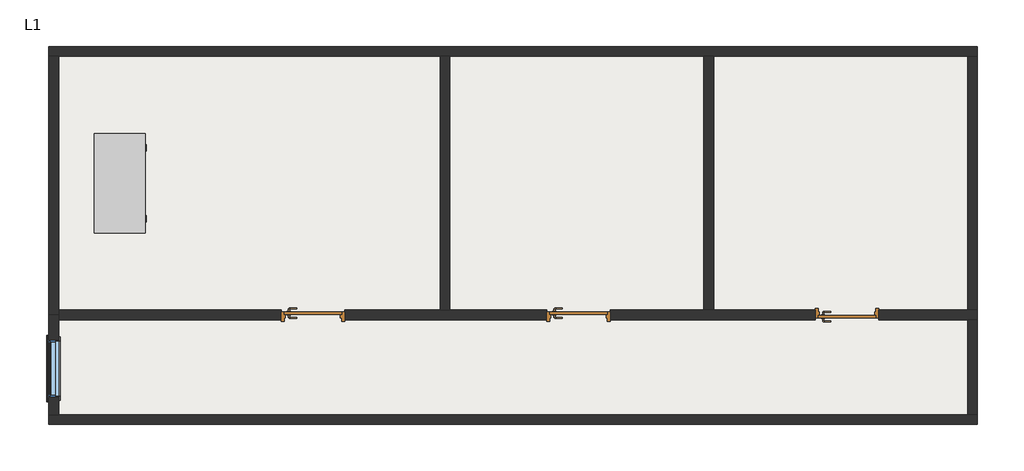
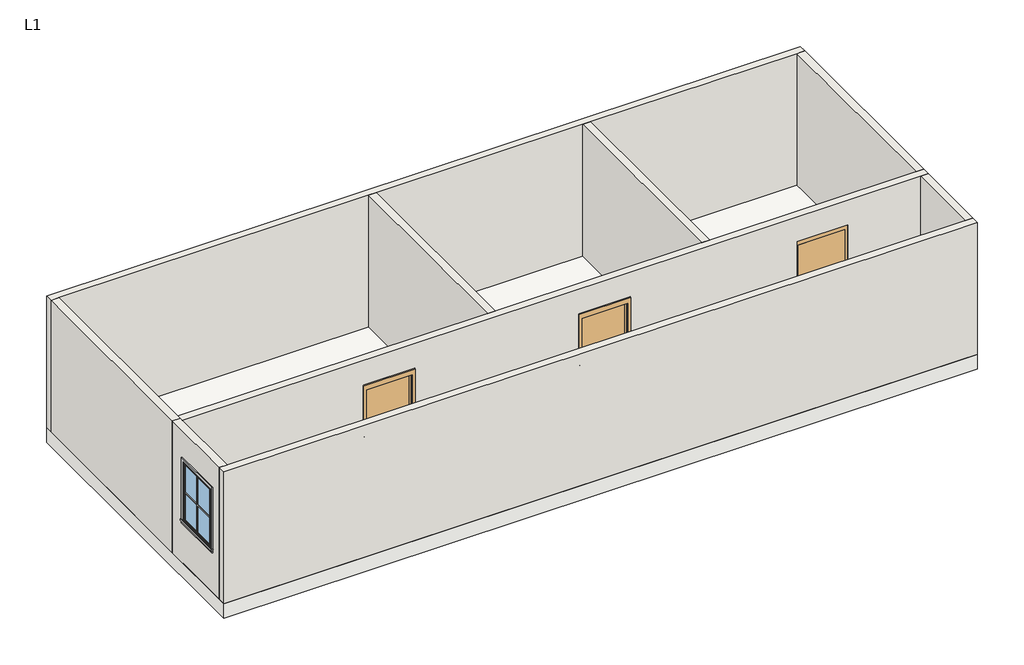
# One storey: 9 walls, 3 doors, 3 proxies, 1 furniture element, 1 slab, 1 window.
"""IFC4 building model written with IfcOpenShell, lengths in millimetres."""

import ifcopenshell
import ifcopenshell.guid

model = None  # the IFC model being written
_history = None  # IfcOwnerHistory: only IFC2X3 demands one
_inside = {}  # id of a spatial element -> (the spatial element, [elements in it])
_under = {}  # id of a project, library or spatial element -> (it, [spatial elements below it])
_declared = {}  # id of a project -> (the project, [libraries it declares])
_typed = {}  # id of a type object -> (the type object, [elements of that type])
_made_of = {}  # id of a material, layer set ... -> (it, [elements and type objects made of it])


def new_model(schema):
    """Start an empty IFC model of exactly this schema.

    Asked for "IFC4X3", IfcOpenShell would pick the latest addendum, in which some entities
    have other attributes; the version numbers below select the first issue.
    IFC2X3 requires an IfcOwnerHistory on every rooted entity: one is made here for all.
    """
    global model, _history
    if schema == "IFC4X3":
        model = ifcopenshell.file(schema_version=(4, 3, 0, 0))
    else:
        model = ifcopenshell.file(schema=schema)
    _inside.clear()
    _under.clear()
    _declared.clear()
    _typed.clear()
    _made_of.clear()
    _history = None
    if model.schema == "IFC2X3":
        org = make("IfcOrganization", Name="unknown")
        user = make(
            "IfcPersonAndOrganization",
            ThePerson=make("IfcPerson", FamilyName="unknown"),
            TheOrganization=org,
        )
        app = make(
            "IfcApplication",
            ApplicationDeveloper=org,
            Version="unknown",
            ApplicationFullName="unknown",
            ApplicationIdentifier="unknown",
        )
        _history = make(
            "IfcOwnerHistory",
            OwningUser=user,
            OwningApplication=app,
            ChangeAction="ADDED",
            CreationDate=0,
        )
    return model


def make(cls, **values):
    """One entity of the class cls with the attributes given. An attribute that is None is left unset."""
    return model.create_entity(
        cls, **{name: value for name, value in values.items() if value is not None}
    )


def rooted(cls, **values):
    """An entity with a GlobalId (a new one), such as an element, a storey or a relation."""
    return make(cls, GlobalId=ifcopenshell.guid.new(), OwnerHistory=_history, **values)


def si_unit(unit_type, name, prefix=None):
    """IfcSIUnit, for example si_unit("LENGTHUNIT", "METRE", prefix="MILLI")."""
    return make("IfcSIUnit", UnitType=unit_type, Prefix=prefix, Name=name)


def assignment(units):
    """IfcUnitAssignment: the units of a project."""
    return None if units is None else make("IfcUnitAssignment", Units=units)


def point(xyz):
    """IfcCartesianPoint."""
    return None if xyz is None else make("IfcCartesianPoint", Coordinates=xyz)


def direction(xyz):
    """IfcDirection."""
    return None if xyz is None else make("IfcDirection", DirectionRatios=xyz)


def frame(location, z_axis=None, x_axis=None):
    """IfcAxis2Placement3D, a coordinate frame: its origin and axes. An axis left out is left unset."""
    return make(
        "IfcAxis2Placement3D",
        Location=point(location),
        Axis=direction(z_axis),
        RefDirection=direction(x_axis),
    )


def frame_2d(location, x_axis=None):
    """IfcAxis2Placement2D, a coordinate frame in the plane: its origin and x axis."""
    return make(
        "IfcAxis2Placement2D", Location=point(location), RefDirection=direction(x_axis)
    )


def origin():
    """The frame at (0, 0, 0) with its axes left unset."""
    return frame((0.0, 0.0, 0.0))


def origin_with_axes():
    """The frame at (0, 0, 0) with the z axis (0, 0, 1) and the x axis (1, 0, 0) written out."""
    return frame((0.0, 0.0, 0.0), z_axis=(0.0, 0.0, 1.0), x_axis=(1.0, 0.0, 0.0))


def place(relative_to, where):
    """IfcLocalPlacement: puts the frame where relative to a parent placement (None: the world)."""
    return make(
        "IfcLocalPlacement", PlacementRelTo=relative_to, RelativePlacement=where
    )


def context(
    kind, dimensions, precision=None, world=None, true_north=None, identifier=None
):
    """IfcGeometricRepresentationContext, for example the 3D "Model" context."""
    return make(
        "IfcGeometricRepresentationContext",
        ContextIdentifier=identifier,
        ContextType=kind,
        CoordinateSpaceDimension=dimensions,
        Precision=precision,
        WorldCoordinateSystem=world,
        TrueNorth=true_north,
    )


def project(units=None, contexts=None):
    """IfcProject with its units and contexts."""
    return rooted(
        "IfcProject",
        Name="project",
        RepresentationContexts=contexts,
        UnitsInContext=assignment(units),
    )


def spatial(cls, under=None, at=None, **own):
    """A site, building, storey or space (cls), placed at a placement, below another one or the project."""
    s = rooted(cls, ObjectPlacement=at, **own)
    if under is not None:
        _under.setdefault(under.id(), (under, []))[1].append(s)
    return s


def polyline(points):
    """IfcPolyline through the points."""
    return make("IfcPolyline", Points=[point(p) for p in points])


def circle_curve(where, radius):
    """IfcCircle in the frame where."""
    return make("IfcCircle", Position=where, Radius=radius)


def ellipse_curve(where, semi_axis1, semi_axis2):
    """IfcEllipse in the frame where."""
    return make(
        "IfcEllipse", Position=where, SemiAxis1=semi_axis1, SemiAxis2=semi_axis2
    )


def trimmed(basis, trim1, trim2, sense, master):
    """IfcTrimmedCurve: the piece of a basis curve between two trims."""
    return make(
        "IfcTrimmedCurve",
        BasisCurve=basis,
        Trim1=trim1,
        Trim2=trim2,
        SenseAgreement=sense,
        MasterRepresentation=master,
    )


def segment(curve, same_sense, transition):
    """IfcCompositeCurveSegment."""
    return make(
        "IfcCompositeCurveSegment",
        Transition=transition,
        SameSense=same_sense,
        ParentCurve=curve,
    )


def composite_curve(segments, self_intersect=None):
    """IfcCompositeCurve: segments joined end to end."""
    return make("IfcCompositeCurve", Segments=segments, SelfIntersect=self_intersect)


def outline(outer, holes=None, kind="AREA"):
    """IfcArbitraryClosedProfileDef: a profile drawn as a closed curve; with holes, ...WithVoids."""
    if holes is None:
        return make("IfcArbitraryClosedProfileDef", ProfileType=kind, OuterCurve=outer)
    return make(
        "IfcArbitraryProfileDefWithVoids",
        ProfileType=kind,
        OuterCurve=outer,
        InnerCurves=holes,
    )


def extrude(swept, where, along, depth):
    """IfcExtrudedAreaSolid: the profile swept, set in the frame where, extruded along a direction by depth."""
    return make(
        "IfcExtrudedAreaSolid",
        SweptArea=swept,
        Position=where,
        ExtrudedDirection=direction(along),
        Depth=depth,
    )


def faces_of(points, faces, orient=None, outer=None):
    """IfcFace entities. A face is a list of loops; a loop is a list of indices into points, from 0.

    orient and outer hold one flag for each loop. By default every Orientation is true, the
    first loop of a face is its IfcFaceOuterBound and the others are IfcFaceBound.
    """
    made = []
    for i, loops in enumerate(faces):
        bounds = []
        for j, loop in enumerate(loops):
            is_outer = j == 0 if outer is None else outer[i][j]
            bounds.append(
                make(
                    "IfcFaceOuterBound" if is_outer else "IfcFaceBound",
                    Bound=make("IfcPolyLoop", Polygon=[points[k] for k in loop]),
                    Orientation=True if orient is None else orient[i][j],
                )
            )
        made.append(make("IfcFace", Bounds=bounds))
    return made


def faceted_brep(points, faces, orient=None, outer=None, voids=None):
    """IfcFacetedBrep: a solid bounded by flat faces; with voids (closed shells), ...WithVoids."""
    shared = [point(p) for p in points]
    hull = make("IfcClosedShell", CfsFaces=faces_of(shared, faces, orient, outer))
    if voids is None:
        return make("IfcFacetedBrep", Outer=hull)
    return make(
        "IfcFacetedBrepWithVoids",
        Outer=hull,
        Voids=[
            make(cls, CfsFaces=faces_of(shared, fs, o, b)) for cls, fs, o, b in voids
        ],
    )


def shape(context_of_items, identifier, shape_type, items):
    """IfcShapeRepresentation: the items that make up one representation, for example the "Body"."""
    return make(
        "IfcShapeRepresentation",
        ContextOfItems=context_of_items,
        RepresentationIdentifier=identifier,
        RepresentationType=shape_type,
        Items=items,
    )


def source(mapping_origin, context_of_items, identifier, shape_type, items):
    """IfcRepresentationMap: a shape defined once, which mapped items show again and again."""
    return make(
        "IfcRepresentationMap",
        MappingOrigin=mapping_origin,
        MappedRepresentation=shape(context_of_items, identifier, shape_type, items),
    )


def transform(
    local_origin,
    x_axis=None,
    y_axis=None,
    z_axis=None,
    scale=None,
    scale2=None,
    scale3=None,
    uniform=True,
):
    """IfcCartesianTransformationOperator3D, or its non-uniform kind. x_axis, y_axis, z_axis: its Axis1, 2, 3."""
    if uniform:
        return make(
            "IfcCartesianTransformationOperator3D",
            Axis1=direction(x_axis),
            Axis2=direction(y_axis),
            LocalOrigin=point(local_origin),
            Scale=scale,
            Axis3=direction(z_axis),
        )
    return make(
        "IfcCartesianTransformationOperator3DnonUniform",
        Axis1=direction(x_axis),
        Axis2=direction(y_axis),
        LocalOrigin=point(local_origin),
        Scale=scale,
        Axis3=direction(z_axis),
        Scale2=scale2,
        Scale3=scale3,
    )


def mapped(mapping_source, mapping_target):
    """IfcMappedItem: shows the shape of a source again, moved by a transform."""
    return make(
        "IfcMappedItem", MappingSource=mapping_source, MappingTarget=mapping_target
    )


def made_of(thing, what):
    """Note that an element or type object is made of a material, layer set ...; save() writes the relation."""
    if what is not None:
        _made_of.setdefault(what.id(), (what, []))[1].append(thing)
    return thing


def element(
    cls,
    number,
    at=None,
    inside=None,
    cuts=None,
    type_object=None,
    material=None,
    context=None,
    identifier="Body",
    shape_type=None,
    held_by="IfcProductDefinitionShape",
    body=None,
    shapes=None,
    **own,
):
    """One element of the class cls, such as IfcWall. Its Tag is "e" and its number.

    at: its placement. inside: the storey or other place that contains it. cuts: it is an
    opening in that element (IfcRelVoidsElement). A single representation is given by context,
    identifier, shape_type and body (its items); several are given by shapes. held_by: the class
    of the entity that holds the representations. save() writes the other relations.
    """
    e = rooted(cls, Tag="e%d" % number, ObjectPlacement=at, **own)
    if body is not None:
        shapes = [shape(context, identifier, shape_type, body)]
    if shapes is not None:
        e.Representation = make(held_by, Representations=shapes)
    if inside is not None:
        _inside.setdefault(inside.id(), (inside, []))[1].append(e)
    if cuts is not None:
        rooted(
            "IfcRelVoidsElement", RelatingBuildingElement=cuts, RelatedOpeningElement=e
        )
    if type_object is not None:
        _typed.setdefault(type_object.id(), (type_object, []))[1].append(e)
    return made_of(e, material)


def aggregate(whole, parts):
    """IfcRelAggregates: a whole, such as a stair, and the parts it consists of."""
    return rooted("IfcRelAggregates", RelatingObject=whole, RelatedObjects=parts)


def save(model, path):
    """Write the relations noted so far, then the file.

    IfcRelAggregates (storeys below a building ...), IfcRelContainedInSpatialStructure (elements
    in a storey), IfcRelDefinesByType, IfcRelAssociatesMaterial and IfcRelDeclares: one each for
    every whole, place, type object, material and project.
    """
    for whole, parts in _under.values():
        aggregate(whole, parts)
    for where, things in _inside.values():
        rooted(
            "IfcRelContainedInSpatialStructure",
            RelatedElements=things,
            RelatingStructure=where,
        )
    for kind, things in _typed.values():
        rooted("IfcRelDefinesByType", RelatedObjects=things, RelatingType=kind)
    for what, things in _made_of.values():
        rooted("IfcRelAssociatesMaterial", RelatedObjects=things, RelatingMaterial=what)
    for by, libraries in _declared.values():
        rooted("IfcRelDeclares", RelatingContext=by, RelatedDefinitions=libraries)
    model.write(path)


def plane_surface(at):
    """IfcPlane: the flat surface through the origin of the frame at, square to its z axis."""
    return make("IfcPlane", Position=at)


def cylinder_surface(at, radius):
    """IfcCylindricalSurface: all points at the distance radius from the z axis of the frame at."""
    return make("IfcCylindricalSurface", Position=at, Radius=radius)


def revolved_surface(curve, axis_point, axis_direction):
    """IfcSurfaceOfRevolution: the curve turned about the line through axis_point along axis_direction."""
    return make(
        "IfcSurfaceOfRevolution",
        SweptCurve=make("IfcArbitraryOpenProfileDef", ProfileType="CURVE", Curve=curve),
        AxisPosition=make("IfcAxis1Placement", Location=point(axis_point), Axis=direction(axis_direction)),
    )


def advanced_brep(points, edges, surfaces, faces):
    """IfcAdvancedBrep: a solid bounded by faces that lie on surfaces and meet in shared edges.

    An edge is (start, end): straight between two places in points (the first is 0);
    or (start, end, curve); or (start, end, curve, False) where it runs against its curve.
    A face is (place in surfaces, loops), or (place, loops, False) where it looks against
    its surface's normal. A loop lists edges by number (the first is 1), with a minus sign
    where the edge is run from its end to its start. The first loop is the outer one.
    """
    corners = [point(p) for p in points]
    vertices = [make("IfcVertexPoint", VertexGeometry=c) for c in corners]
    made = []
    for start, end, *more in edges:
        made.append(
            make(
                "IfcEdgeCurve",
                EdgeStart=vertices[start],
                EdgeEnd=vertices[end],
                EdgeGeometry=more[0] if more else make("IfcPolyline", Points=[corners[start], corners[end]]),
                SameSense=more[1] if len(more) > 1 else True,
            )
        )
    hull = []
    for where, loops, *sense in faces:
        bounds = []
        for j, loop in enumerate(loops):
            ring = [make("IfcOrientedEdge", EdgeElement=made[abs(k) - 1], Orientation=k > 0) for k in loop]
            bounds.append(
                make(
                    "IfcFaceOuterBound" if j == 0 else "IfcFaceBound",
                    Bound=make("IfcEdgeLoop", EdgeList=ring),
                    Orientation=True,
                )
            )
        hull.append(make("IfcAdvancedFace", Bounds=bounds, FaceSurface=surfaces[where], SameSense=sense[0] if sense else True))
    return make("IfcAdvancedBrep", Outer=make("IfcClosedShell", CfsFaces=hull))


def m_muntin_pattern_2x2_m_muntin_pattern_2x2_ad852c99(model_context):
    return source(origin(), model_context, "Body", "SweptSolid", [
        extrude(outline(polyline([(568.25, -6.35), (568.25, -411.9), (555.55, -411.9), (555.55, -6.35), (0.0, -6.35), (0.0, 6.35), (555.55, 6.35), (555.55, 411.9), (568.25, 411.9), (568.25, 6.35), (1123.8, 6.35), (1123.8, -6.35), (568.25, -6.35)])), frame((0.0, -22.225, 0.0), z_axis=(0.0, 1.0, 0.0), x_axis=(0.0, 0.0, 1.0)), (0.0, 0.0, 1.0), 12.7),
        extrude(outline(polyline([(568.25, -6.35), (568.25, -411.9), (555.55, -411.9), (555.55, -6.35), (0.0, -6.35), (0.0, 6.35), (555.55, 6.35), (555.55, 411.9), (568.25, 411.9), (568.25, 6.35), (1123.8, 6.35), (1123.8, -6.35), (568.25, -6.35)])), frame((0.0, 9.525, 0.0), z_axis=(0.0, 1.0, 0.0), x_axis=(0.0, 0.0, 1.0)), (0.0, 0.0, 1.0), 12.7),
    ])


def m_trim_window_exterior_flat_with_sill_71544b40(model_context):
    return source(origin(), model_context, "Body", "SweptSolid", [
        extrude(outline(polyline([(510.0, -1220.4323709), (510.0, -1280.4323709), (-510.0, -1280.4323709), (-510.0, -1220.4323709), (510.0, -1220.4323709)])), origin_with_axes(), (0.0, 0.0, 1.0), 19.05),
        extrude(outline(polyline([(-1230.0, 38.1), (-1202.4580645, 38.1), (-1200.0, 19.05), (-1200.0, 0.0), (-1220.4323709, 0.0), (-1220.4323709, 19.05), (-1230.0, 19.05), (-1230.0, 38.1)])), frame((-522.7, 0.0, 0.0), z_axis=(1.0, 0.0, 0.0), x_axis=(0.0, 1.0, 0.0)), (0.0, 0.0, 1.0), 1045.4),
        extrude(outline(polyline([(-510.0, 60.0), (510.0, 60.0), (510.0, -1200.0), (450.0, -1200.0), (450.0, 0.0), (-450.0, 0.0), (-450.0, -1200.0), (-510.0, -1200.0), (-510.0, 60.0)])), origin_with_axes(), (0.0, 0.0, 1.0), 19.05),
    ])


def m_trim_window_interior_flat_picture_frame_24fe8ef8(model_context):
    return source(origin(), model_context, "Body", "SweptSolid", [
        extrude(outline(polyline([(497.3, 47.3), (497.3, -1247.3), (-497.3, -1247.3), (-497.3, 47.3), (497.3, 47.3)]), holes=[polyline([(437.3, -12.7), (-437.3, -12.7), (-437.3, -1187.3), (437.3, -1187.3), (437.3, -12.7)])]), origin_with_axes(), (0.0, 0.0, 1.0), 30.0),
    ])


def m_door_passage_single_flush_900_x_2100mm_f70d95c9(model_context):
    return source(origin(), model_context, "Body", "SolidModel", [
        advanced_brep(
        [(-384.990625, 3.35, 1000.0), (-364.990625, 3.35, 1000.0), (-364.990625, -26.65, 1000.0), (-384.990625, -26.65, 1000.0), (-359.990625, -31.65, 1000.0), (-359.990625, -51.65, 1000.0), (-254.990625, -51.65, 1000.0), (-254.990625, -31.65, 1000.0)],
        [
            (0, 1, circle_curve(frame((-374.990625, 3.35, 1000.0), z_axis=(0.0, 1.0, 0.0), x_axis=(1.0, 0.0, 0.0)), 10.0)),
            (1, 0, circle_curve(frame((-374.990625, 3.35, 1000.0), z_axis=(0.0, 1.0, 0.0), x_axis=(1.0, 0.0, 0.0)), 10.0)),
            (1, 2),
            (2, 3, circle_curve(frame((-374.990625, -26.65, 1000.0), z_axis=(0.0, 1.0, 0.0), x_axis=(1.0, 0.0, 0.0)), 10.0)),
            (3, 0),
            (3, 2, circle_curve(frame((-374.990625, -26.65, 1000.0), z_axis=(0.0, 1.0, 0.0), x_axis=(1.0, 0.0, 0.0)), 10.0)),
            (4, 5, circle_curve(frame((-359.990625, -41.65, 1000.0), z_axis=(-1.0, 0.0, 0.0), x_axis=(0.0, 1.0, 0.0)), 10.0)),
            (5, 3, circle_curve(frame((-359.990625, -26.65, 1000.0), z_axis=(0.0, 0.0, -1.0), x_axis=(-1.0, 0.0, 0.0)), 25.0)),
            (2, 4, circle_curve(frame((-359.990625, -26.65, 1000.0), z_axis=(0.0, 0.0, 1.0), x_axis=(-1.0, 0.0, 0.0)), 5.0)),
            (5, 4, circle_curve(frame((-359.990625, -41.65, 1000.0), z_axis=(-1.0, 0.0, 0.0), x_axis=(0.0, 1.0, 0.0)), 10.0)),
            (6, 7, circle_curve(frame((-254.990625, -41.65, 1000.0), z_axis=(1.0, 0.0, 0.0), x_axis=(0.0, 1.0, 0.0)), 10.0)),
            (7, 6, circle_curve(frame((-254.990625, -41.65, 1000.0), z_axis=(1.0, 0.0, 0.0), x_axis=(0.0, 1.0, 0.0)), 10.0)),
            (4, 7),
            (6, 5),
        ],
        [
            plane_surface(frame((-374.990625, 3.35, 1000.0), z_axis=(0.0, 1.0, 0.0), x_axis=(0.0, 0.0, 1.0))),
            cylinder_surface(frame((-374.990625, 3.35, 1000.0), z_axis=(0.0, 1.0, 0.0), x_axis=(1.0, 0.0, 0.0)), 10.0),
            revolved_surface(trimmed(ellipse_curve(frame((-374.990625, -26.65, 1000.0), z_axis=(0.0, -1.0, 0.0), x_axis=(1.0, 0.0, 0.0)), 10.0, 10.0), [point((-384.990625, -26.65, 1000.0))], [point((-364.990625, -26.65, 1000.0))], True, "CARTESIAN"), (-359.990625, -26.65, 1000.0), (0.0, 0.0, -1.0)),
            revolved_surface(trimmed(ellipse_curve(frame((-374.990625, -26.65, 1000.0), z_axis=(0.0, -1.0, 0.0), x_axis=(1.0, 0.0, 0.0)), 10.0, 10.0), [point((-364.990625, -26.65, 1000.0))], [point((-384.990625, -26.65, 1000.0))], True, "CARTESIAN"), (-359.990625, -26.65, 1000.0), (0.0, 0.0, -1.0)),
            plane_surface(frame((-254.990625, -41.65, 1000.0), z_axis=(1.0, 0.0, 0.0), x_axis=(0.0, 0.0, 1.0))),
            cylinder_surface(frame((-359.990625, -41.65, 1000.0), z_axis=(-1.0, 0.0, 0.0), x_axis=(0.0, 1.0, 0.0)), 10.0),
        ],
        [
            (0, [[1, 2]]),
            (1, [[3, 4, 5, -2]]),
            (1, [[-5, 6, -3, -1]]),
            (2, [[7, 8, -4, 9]]),
            (3, [[10, -9, -6, -8]]),
            (4, [[11, 12]]),
            (5, [[13, -11, 14, -7]]),
            (5, [[-14, -12, -13, -10]]),
        ],
    ),
        extrude(outline(composite_curve([segment(trimmed(circle_curve(frame_2d((1000.0, -377.490625)), 30.0), [point((1000.0, -407.490625))], [point((1000.0, -347.490625))], False, "CARTESIAN"), True, "CONTINUOUS"), segment(trimmed(circle_curve(frame_2d((1000.0, -377.490625)), 30.0), [point((1000.0, -347.490625))], [point((1000.0, -407.490625))], False, "CARTESIAN"), True, "CONTINUOUS")], self_intersect=False)), frame((0.0, 3.35, 0.0), z_axis=(0.0, 1.0, 0.0), x_axis=(0.0, 0.0, 1.0)), (0.0, 0.0, 1.0), 8.0),
        advanced_brep(
        [(-384.990625, 64.35, 1000.0), (-364.990625, 64.35, 1000.0), (-384.990625, 94.35, 1000.0), (-364.990625, 94.35, 1000.0), (-359.990625, 99.35, 1000.0), (-359.990625, 119.35, 1000.0), (-254.990625, 119.35, 1000.0), (-254.990625, 99.35, 1000.0)],
        [
            (0, 1, circle_curve(frame((-374.990625, 64.35, 1000.0), z_axis=(0.0, -1.0, 0.0), x_axis=(1.0, 0.0, 0.0)), 10.0)),
            (1, 0, circle_curve(frame((-374.990625, 64.35, 1000.0), z_axis=(0.0, -1.0, 0.0), x_axis=(1.0, 0.0, 0.0)), 10.0)),
            (0, 2),
            (2, 3, circle_curve(frame((-374.990625, 94.35, 1000.0), z_axis=(0.0, -1.0, 0.0), x_axis=(1.0, 0.0, 0.0)), 10.0)),
            (3, 1),
            (3, 2, circle_curve(frame((-374.990625, 94.35, 1000.0), z_axis=(0.0, -1.0, 0.0), x_axis=(1.0, 0.0, 0.0)), 10.0)),
            (4, 3, circle_curve(frame((-359.990625, 94.35, 1000.0), z_axis=(0.0, 0.0, 1.0), x_axis=(-1.0, 0.0, 0.0)), 5.0)),
            (2, 5, circle_curve(frame((-359.990625, 94.35, 1000.0), z_axis=(0.0, 0.0, -1.0), x_axis=(-1.0, 0.0, 0.0)), 25.0)),
            (5, 4, circle_curve(frame((-359.990625, 109.35, 1000.0), z_axis=(-1.0, 0.0, 0.0), x_axis=(0.0, -1.0, 0.0)), 10.0)),
            (4, 5, circle_curve(frame((-359.990625, 109.35, 1000.0), z_axis=(-1.0, 0.0, 0.0), x_axis=(0.0, -1.0, 0.0)), 10.0)),
            (6, 7, circle_curve(frame((-254.990625, 109.35, 1000.0), z_axis=(1.0, 0.0, 0.0), x_axis=(0.0, -1.0, 0.0)), 10.0)),
            (7, 6, circle_curve(frame((-254.990625, 109.35, 1000.0), z_axis=(1.0, 0.0, 0.0), x_axis=(0.0, -1.0, 0.0)), 10.0)),
            (5, 6),
            (7, 4),
        ],
        [
            plane_surface(frame((-374.990625, 64.35, 1000.0), z_axis=(0.0, -1.0, 0.0), x_axis=(0.0, 0.0, 1.0))),
            cylinder_surface(frame((-374.990625, 64.35, 1000.0), z_axis=(0.0, -1.0, 0.0), x_axis=(1.0, 0.0, 0.0)), 10.0),
            revolved_surface(trimmed(ellipse_curve(frame((-374.990625, 94.35, 1000.0), z_axis=(0.0, -1.0, 0.0), x_axis=(1.0, 0.0, 0.0)), 10.0, 10.0), [point((-384.990625, 94.35, 1000.0))], [point((-364.990625, 94.35, 1000.0))], True, "CARTESIAN"), (-359.990625, 94.35, 1000.0), (0.0, 0.0, -1.0)),
            revolved_surface(trimmed(ellipse_curve(frame((-374.990625, 94.35, 1000.0), z_axis=(0.0, -1.0, 0.0), x_axis=(1.0, 0.0, 0.0)), 10.0, 10.0), [point((-364.990625, 94.35, 1000.0))], [point((-384.990625, 94.35, 1000.0))], True, "CARTESIAN"), (-359.990625, 94.35, 1000.0), (0.0, 0.0, -1.0)),
            plane_surface(frame((-254.990625, 109.35, 1000.0), z_axis=(1.0, 0.0, 0.0), x_axis=(0.0, 0.0, 1.0))),
            cylinder_surface(frame((-359.990625, 109.35, 1000.0), z_axis=(-1.0, 0.0, 0.0), x_axis=(0.0, -1.0, 0.0)), 10.0),
        ],
        [
            (0, [[1, 2]]),
            (1, [[-1, 3, 4, 5]]),
            (1, [[-2, -5, 6, -3]]),
            (2, [[7, -4, 8, 9]]),
            (3, [[-8, -6, -7, 10]]),
            (4, [[11, 12]]),
            (5, [[-9, 13, -12, 14]]),
            (5, [[-10, -14, -11, -13]]),
        ],
    ),
        extrude(outline(composite_curve([segment(trimmed(circle_curve(frame_2d((1000.0, -377.490625)), 30.0), [point((1000.0, -407.490625))], [point((1000.0, -347.490625))], False, "CARTESIAN"), True, "CONTINUOUS"), segment(trimmed(circle_curve(frame_2d((1000.0, -377.490625)), 30.0), [point((1000.0, -347.490625))], [point((1000.0, -407.490625))], False, "CARTESIAN"), True, "CONTINUOUS")], self_intersect=False)), frame((0.0, 56.35, 0.0), z_axis=(0.0, 1.0, 0.0), x_axis=(0.0, 0.0, 1.0)), (0.0, 0.0, 1.0), 8.0),
        extrude(outline(polyline([(450.0, 11.35), (-450.0, 11.35), (-450.0, 56.35), (450.0, 56.35), (450.0, 11.35)])), origin_with_axes(), (0.0, 0.0, 1.0), 2100.0),
        faceted_brep([(450.0, 6.5875, 0.0), (450.0, 56.35, 0.0), (500.0, 56.35, 0.0), (500.0, -93.65, 0.0), (450.0, -93.65, 0.0), (450.0, -44.4375, 0.0), (434.125, -44.4375, 0.0), (434.125, 6.5875, 0.0), (450.0, 6.5875, 2100.0), (450.0, 56.35, 2100.0), (-450.0, 56.35, 2100.0), (-450.0, 56.35, 0.0), (-500.0, 56.35, 0.0), (-500.0, 56.35, 2200.0), (500.0, 56.35, 2200.0), (500.0, -93.65, 2200.0), (-500.0, -93.65, 2200.0), (-500.0, -93.65, 0.0), (-450.0, -93.65, 0.0), (-450.0, -93.65, 2100.0), (450.0, -93.65, 2100.0), (450.0, -44.4375, 2100.0), (-450.0, -44.4375, 2100.0), (-450.0, -44.4375, 0.0), (-434.125, -44.4375, 0.0), (-434.125, -44.4375, 2084.125), (434.125, -44.4375, 2084.125), (434.125, 6.5875, 2084.125), (-434.125, 6.5875, 2084.125), (-434.125, 6.5875, 0.0), (-450.0, 6.5875, 0.0), (-450.0, 6.5875, 2100.0)], [[[0, 1, 2, 3, 4, 5, 6, 7]], [[1, 0, 8, 9]], [[2, 1, 9, 10, 11, 12, 13, 14]], [[3, 2, 14, 15]], [[4, 3, 15, 16, 17, 18, 19, 20]], [[5, 4, 20, 21]], [[6, 5, 21, 22, 23, 24, 25, 26]], [[7, 6, 26, 27]], [[0, 7, 27, 28, 29, 30, 31, 8]], [[9, 8, 31, 10]], [[20, 19, 22, 21]], [[26, 25, 28, 27]], [[12, 11, 30, 29, 24, 23, 18, 17]], [[11, 10, 31, 30]], [[13, 12, 17, 16]], [[19, 18, 23, 22]], [[25, 24, 29, 28]], [[15, 14, 13, 16]]]),
    ])


def m_door_passage_single_flush_900_x_2100mm_89322b7b(model_context):
    return source(origin(), model_context, "Body", "SolidModel", [
        advanced_brep(
        [(-384.990625, -3.35, 1000.0), (-364.990625, -3.35, 1000.0), (-384.990625, 26.65, 1000.0), (-364.990625, 26.65, 1000.0), (-359.990625, 31.65, 1000.0), (-359.990625, 51.65, 1000.0), (-254.990625, 51.65, 1000.0), (-254.990625, 31.65, 1000.0)],
        [
            (0, 1, circle_curve(frame((-374.990625, -3.35, 1000.0), z_axis=(0.0, -1.0, 0.0), x_axis=(1.0, 0.0, 0.0)), 10.0)),
            (1, 0, circle_curve(frame((-374.990625, -3.35, 1000.0), z_axis=(0.0, -1.0, 0.0), x_axis=(1.0, 0.0, 0.0)), 10.0)),
            (0, 2),
            (2, 3, circle_curve(frame((-374.990625, 26.65, 1000.0), z_axis=(0.0, -1.0, 0.0), x_axis=(1.0, 0.0, 0.0)), 10.0)),
            (3, 1),
            (3, 2, circle_curve(frame((-374.990625, 26.65, 1000.0), z_axis=(0.0, -1.0, 0.0), x_axis=(1.0, 0.0, 0.0)), 10.0)),
            (4, 3, circle_curve(frame((-359.990625, 26.65, 1000.0), z_axis=(0.0, 0.0, 1.0), x_axis=(-1.0, 0.0, 0.0)), 5.0)),
            (2, 5, circle_curve(frame((-359.990625, 26.65, 1000.0), z_axis=(0.0, 0.0, -1.0), x_axis=(-1.0, 0.0, 0.0)), 25.0)),
            (5, 4, circle_curve(frame((-359.990625, 41.65, 1000.0), z_axis=(-1.0, 0.0, 0.0), x_axis=(0.0, -1.0, 0.0)), 10.0)),
            (4, 5, circle_curve(frame((-359.990625, 41.65, 1000.0), z_axis=(-1.0, 0.0, 0.0), x_axis=(0.0, -1.0, 0.0)), 10.0)),
            (6, 7, circle_curve(frame((-254.990625, 41.65, 1000.0), z_axis=(1.0, 0.0, 0.0), x_axis=(0.0, -1.0, 0.0)), 10.0)),
            (7, 6, circle_curve(frame((-254.990625, 41.65, 1000.0), z_axis=(1.0, 0.0, 0.0), x_axis=(0.0, -1.0, 0.0)), 10.0)),
            (5, 6),
            (7, 4),
        ],
        [
            plane_surface(frame((-374.990625, -3.35, 1000.0), z_axis=(0.0, -1.0, 0.0), x_axis=(0.0, 0.0, 1.0))),
            cylinder_surface(frame((-374.990625, -3.35, 1000.0), z_axis=(0.0, -1.0, 0.0), x_axis=(1.0, 0.0, 0.0)), 10.0),
            revolved_surface(trimmed(ellipse_curve(frame((-374.990625, 26.65, 1000.0), z_axis=(0.0, -1.0, 0.0), x_axis=(1.0, 0.0, 0.0)), 10.0, 10.0), [point((-384.990625, 26.65, 1000.0))], [point((-364.990625, 26.65, 1000.0))], True, "CARTESIAN"), (-359.990625, 26.65, 1000.0), (0.0, 0.0, -1.0)),
            revolved_surface(trimmed(ellipse_curve(frame((-374.990625, 26.65, 1000.0), z_axis=(0.0, -1.0, 0.0), x_axis=(1.0, 0.0, 0.0)), 10.0, 10.0), [point((-364.990625, 26.65, 1000.0))], [point((-384.990625, 26.65, 1000.0))], True, "CARTESIAN"), (-359.990625, 26.65, 1000.0), (0.0, 0.0, -1.0)),
            plane_surface(frame((-254.990625, 41.65, 1000.0), z_axis=(1.0, 0.0, 0.0), x_axis=(0.0, 0.0, 1.0))),
            cylinder_surface(frame((-359.990625, 41.65, 1000.0), z_axis=(-1.0, 0.0, 0.0), x_axis=(0.0, -1.0, 0.0)), 10.0),
        ],
        [
            (0, [[1, 2]]),
            (1, [[-1, 3, 4, 5]]),
            (1, [[-2, -5, 6, -3]]),
            (2, [[7, -4, 8, 9]]),
            (3, [[-8, -6, -7, 10]]),
            (4, [[11, 12]]),
            (5, [[-9, 13, -12, 14]]),
            (5, [[-10, -14, -11, -13]]),
        ],
    ),
        extrude(outline(composite_curve([segment(trimmed(circle_curve(frame_2d((1000.0, -377.490625)), 30.0), [point((1000.0, -407.490625))], [point((1000.0, -347.490625))], False, "CARTESIAN"), True, "CONTINUOUS"), segment(trimmed(circle_curve(frame_2d((1000.0, -377.490625)), 30.0), [point((1000.0, -347.490625))], [point((1000.0, -407.490625))], False, "CARTESIAN"), True, "CONTINUOUS")], self_intersect=False)), frame((0.0, -11.35, 0.0), z_axis=(0.0, 1.0, 0.0), x_axis=(0.0, 0.0, 1.0)), (0.0, 0.0, 1.0), 8.0),
        advanced_brep(
        [(-384.990625, -64.35, 1000.0), (-364.990625, -64.35, 1000.0), (-364.990625, -94.35, 1000.0), (-384.990625, -94.35, 1000.0), (-359.990625, -99.35, 1000.0), (-359.990625, -119.35, 1000.0), (-254.990625, -119.35, 1000.0), (-254.990625, -99.35, 1000.0)],
        [
            (0, 1, circle_curve(frame((-374.990625, -64.35, 1000.0), z_axis=(0.0, 1.0, 0.0), x_axis=(1.0, 0.0, 0.0)), 10.0)),
            (1, 0, circle_curve(frame((-374.990625, -64.35, 1000.0), z_axis=(0.0, 1.0, 0.0), x_axis=(1.0, 0.0, 0.0)), 10.0)),
            (1, 2),
            (2, 3, circle_curve(frame((-374.990625, -94.35, 1000.0), z_axis=(0.0, 1.0, 0.0), x_axis=(1.0, 0.0, 0.0)), 10.0)),
            (3, 0),
            (3, 2, circle_curve(frame((-374.990625, -94.35, 1000.0), z_axis=(0.0, 1.0, 0.0), x_axis=(1.0, 0.0, 0.0)), 10.0)),
            (4, 5, circle_curve(frame((-359.990625, -109.35, 1000.0), z_axis=(-1.0, 0.0, 0.0), x_axis=(0.0, 1.0, 0.0)), 10.0)),
            (5, 3, circle_curve(frame((-359.990625, -94.35, 1000.0), z_axis=(0.0, 0.0, -1.0), x_axis=(-1.0, 0.0, 0.0)), 25.0)),
            (2, 4, circle_curve(frame((-359.990625, -94.35, 1000.0), z_axis=(0.0, 0.0, 1.0), x_axis=(-1.0, 0.0, 0.0)), 5.0)),
            (5, 4, circle_curve(frame((-359.990625, -109.35, 1000.0), z_axis=(-1.0, 0.0, 0.0), x_axis=(0.0, 1.0, 0.0)), 10.0)),
            (6, 7, circle_curve(frame((-254.990625, -109.35, 1000.0), z_axis=(1.0, 0.0, 0.0), x_axis=(0.0, 1.0, 0.0)), 10.0)),
            (7, 6, circle_curve(frame((-254.990625, -109.35, 1000.0), z_axis=(1.0, 0.0, 0.0), x_axis=(0.0, 1.0, 0.0)), 10.0)),
            (4, 7),
            (6, 5),
        ],
        [
            plane_surface(frame((-374.990625, -64.35, 1000.0), z_axis=(0.0, 1.0, 0.0), x_axis=(0.0, 0.0, 1.0))),
            cylinder_surface(frame((-374.990625, -64.35, 1000.0), z_axis=(0.0, 1.0, 0.0), x_axis=(1.0, 0.0, 0.0)), 10.0),
            revolved_surface(trimmed(ellipse_curve(frame((-374.990625, -94.35, 1000.0), z_axis=(0.0, -1.0, 0.0), x_axis=(1.0, 0.0, 0.0)), 10.0, 10.0), [point((-384.990625, -94.35, 1000.0))], [point((-364.990625, -94.35, 1000.0))], True, "CARTESIAN"), (-359.990625, -94.35, 1000.0), (0.0, 0.0, -1.0)),
            revolved_surface(trimmed(ellipse_curve(frame((-374.990625, -94.35, 1000.0), z_axis=(0.0, -1.0, 0.0), x_axis=(1.0, 0.0, 0.0)), 10.0, 10.0), [point((-364.990625, -94.35, 1000.0))], [point((-384.990625, -94.35, 1000.0))], True, "CARTESIAN"), (-359.990625, -94.35, 1000.0), (0.0, 0.0, -1.0)),
            plane_surface(frame((-254.990625, -109.35, 1000.0), z_axis=(1.0, 0.0, 0.0), x_axis=(0.0, 0.0, 1.0))),
            cylinder_surface(frame((-359.990625, -109.35, 1000.0), z_axis=(-1.0, 0.0, 0.0), x_axis=(0.0, 1.0, 0.0)), 10.0),
        ],
        [
            (0, [[1, 2]]),
            (1, [[3, 4, 5, -2]]),
            (1, [[-5, 6, -3, -1]]),
            (2, [[7, 8, -4, 9]]),
            (3, [[10, -9, -6, -8]]),
            (4, [[11, 12]]),
            (5, [[13, -11, 14, -7]]),
            (5, [[-14, -12, -13, -10]]),
        ],
    ),
        extrude(outline(composite_curve([segment(trimmed(circle_curve(frame_2d((1000.0, -377.490625)), 30.0), [point((1000.0, -407.490625))], [point((1000.0, -347.490625))], False, "CARTESIAN"), True, "CONTINUOUS"), segment(trimmed(circle_curve(frame_2d((1000.0, -377.490625)), 30.0), [point((1000.0, -347.490625))], [point((1000.0, -407.490625))], False, "CARTESIAN"), True, "CONTINUOUS")], self_intersect=False)), frame((0.0, -64.35, 0.0), z_axis=(0.0, 1.0, 0.0), x_axis=(0.0, 0.0, 1.0)), (0.0, 0.0, 1.0), 8.0),
        extrude(outline(polyline([(450.0, -11.35), (450.0, -56.35), (-450.0, -56.35), (-450.0, -11.35), (450.0, -11.35)])), origin_with_axes(), (0.0, 0.0, 1.0), 2100.0),
        faceted_brep([(450.0, -6.5875, 0.0), (434.125, -6.5875, 0.0), (434.125, 44.4375, 0.0), (450.0, 44.4375, 0.0), (450.0, 93.65, 0.0), (500.0, 93.65, 0.0), (500.0, -56.35, 0.0), (450.0, -56.35, 0.0), (450.0, -56.35, 2100.0), (450.0, -6.5875, 2100.0), (500.0, -56.35, 2200.0), (-500.0, -56.35, 2200.0), (-500.0, -56.35, 0.0), (-450.0, -56.35, 0.0), (-450.0, -56.35, 2100.0), (500.0, 93.65, 2200.0), (450.0, 93.65, 2100.0), (-450.0, 93.65, 2100.0), (-450.0, 93.65, 0.0), (-500.0, 93.65, 0.0), (-500.0, 93.65, 2200.0), (450.0, 44.4375, 2100.0), (434.125, 44.4375, 2084.125), (-434.125, 44.4375, 2084.125), (-434.125, 44.4375, 0.0), (-450.0, 44.4375, 0.0), (-450.0, 44.4375, 2100.0), (434.125, -6.5875, 2084.125), (-450.0, -6.5875, 2100.0), (-450.0, -6.5875, 0.0), (-434.125, -6.5875, 0.0), (-434.125, -6.5875, 2084.125)], [[[0, 1, 2, 3, 4, 5, 6, 7]], [[7, 8, 9, 0]], [[6, 10, 11, 12, 13, 14, 8, 7]], [[5, 15, 10, 6]], [[4, 16, 17, 18, 19, 20, 15, 5]], [[3, 21, 16, 4]], [[2, 22, 23, 24, 25, 26, 21, 3]], [[1, 27, 22, 2]], [[0, 9, 28, 29, 30, 31, 27, 1]], [[8, 14, 28, 9]], [[16, 21, 26, 17]], [[22, 27, 31, 23]], [[12, 19, 18, 25, 24, 30, 29, 13]], [[13, 29, 28, 14]], [[11, 20, 19, 12]], [[17, 26, 25, 18]], [[23, 31, 30, 24]], [[15, 20, 11, 10]]]),
    ])


def m_desk_1525_x_762mm_student_34485ced(model_context):
    return source(origin(), model_context, "Body", "SolidModel", [
        extrude(outline(polyline([(1118.1, 0.0), (1118.1, 635.0), (405.9, 635.0), (405.9, 0.0), (-0.5, 0.0), (-0.5, 762.0), (1524.5, 762.0), (1524.5, 0.0), (1118.1, 0.0)])), frame((0.0, 0.0, 152.0), z_axis=(0.0, 0.0, 1.0), x_axis=(1.0, 0.0, 0.0)), (0.0, 0.0, 1.0), 571.9),
        extrude(outline(polyline([(-19.55, -19.05), (-19.55, 781.05), (1543.55, 781.05), (1543.55, -19.05), (-19.55, -19.05)])), frame((0.0, 0.0, 723.9), z_axis=(0.0, 0.0, 1.0), x_axis=(1.0, 0.0, 0.0)), (0.0, 0.0, 1.0), 38.1),
        faceted_brep([(1422.9, 0.0, 152.0), (1524.5, 0.0, 152.0), (1524.5, 101.6, 152.0), (1422.9, 101.6, 152.0), (1448.3, 0.0, 0.0), (1448.3, 76.2, 0.0), (1524.5, 76.2, 0.0), (1524.5, 0.0, 0.0)], [[[0, 1, 2, 3]], [[4, 5, 6, 7]], [[4, 7, 1, 0]], [[7, 6, 2, 1]], [[6, 5, 3, 2]], [[5, 4, 0, 3]]]),
        faceted_brep([(1422.9, 762.0, 152.0), (1422.9, 660.4, 152.0), (1524.5, 660.4, 152.0), (1524.5, 762.0, 152.0), (1448.3, 762.0, 0.0), (1524.5, 762.0, 0.0), (1524.5, 685.8, 0.0), (1448.3, 685.8, 0.0)], [[[0, 1, 2, 3]], [[4, 5, 6, 7]], [[4, 7, 1, 0]], [[7, 6, 2, 1]], [[6, 5, 3, 2]], [[5, 4, 0, 3]]]),
        faceted_brep([(101.1, 762.0, 152.0), (-0.5, 762.0, 152.0), (-0.5, 660.4, 152.0), (101.1, 660.4, 152.0), (75.7, 762.0, 0.0), (75.7, 685.8, 0.0), (-0.5, 685.8, 0.0), (-0.5, 762.0, 0.0)], [[[0, 1, 2, 3]], [[4, 5, 6, 7]], [[4, 7, 1, 0]], [[7, 6, 2, 1]], [[6, 5, 3, 2]], [[5, 4, 0, 3]]]),
        faceted_brep([(101.1, 0.0, 152.0), (101.1, 101.6, 152.0), (-0.5, 101.6, 152.0), (-0.5, 0.0, 152.0), (75.7, 0.0, 0.0), (-0.5, 0.0, 0.0), (-0.5, 76.2, 0.0), (75.7, 76.2, 0.0)], [[[0, 1, 2, 3]], [[4, 5, 6, 7]], [[4, 7, 1, 0]], [[7, 6, 2, 1]], [[6, 5, 3, 2]], [[5, 4, 0, 3]]]),
        extrude(outline(polyline([(1137.15, 0.0), (1505.45, 0.0), (1505.45, -12.7), (1137.15, -12.7), (1137.15, 0.0)])), frame((0.0, 0.0, 602.85), z_axis=(0.0, 0.0, 1.0), x_axis=(1.0, 0.0, 0.0)), (0.0, 0.0, 1.0), 102.0),
        extrude(outline(polyline([(1137.15, 0.0), (1505.45, 0.0), (1505.45, -12.7), (1137.15, -12.7), (1137.15, 0.0)])), frame((0.0, 0.0, 171.05), z_axis=(0.0, 0.0, 1.0), x_axis=(1.0, 0.0, 0.0)), (0.0, 0.0, 1.0), 171.45),
        extrude(outline(polyline([(1137.15, 0.0), (1505.45, 0.0), (1505.45, -12.7), (1137.15, -12.7), (1137.15, 0.0)])), frame((0.0, 0.0, 482.2), z_axis=(0.0, 0.0, 1.0), x_axis=(1.0, 0.0, 0.0)), (0.0, 0.0, 1.0), 101.6),
        extrude(outline(polyline([(1137.15, 0.0), (1505.45, 0.0), (1505.45, -12.7), (1137.15, -12.7), (1137.15, 0.0)])), frame((0.0, 0.0, 361.55), z_axis=(0.0, 0.0, 1.0), x_axis=(1.0, 0.0, 0.0)), (0.0, 0.0, 1.0), 101.6),
        extrude(outline(polyline([(18.55, 0.0), (386.85, 0.0), (386.85, -12.7), (18.55, -12.7), (18.55, 0.0)])), frame((0.0, 0.0, 603.25), z_axis=(0.0, 0.0, 1.0), x_axis=(1.0, 0.0, 0.0)), (0.0, 0.0, 1.0), 101.6),
        extrude(outline(polyline([(18.55, 0.0), (386.85, 0.0), (386.85, -12.7), (18.55, -12.7), (18.55, 0.0)])), frame((0.0, 0.0, 171.05), z_axis=(0.0, 0.0, 1.0), x_axis=(1.0, 0.0, 0.0)), (0.0, 0.0, 1.0), 413.15),
        faceted_brep([(1365.75, -12.7, 304.8), (1372.1, -12.7, 304.8), (1372.1, -12.7, 292.1), (1365.75, -12.7, 292.1), (1365.75, -31.75, 304.8), (1372.1, -38.1, 304.8), (1372.1, -38.1, 292.1), (1365.75, -31.75, 292.1), (1276.85, -31.75, 304.8), (1270.5, -38.1, 304.8), (1270.5, -38.1, 292.1), (1276.85, -31.75, 292.1), (1276.85, -12.7, 304.8), (1276.85, -12.7, 292.1), (1270.5, -12.7, 292.1), (1270.5, -12.7, 304.8)], [[[0, 1, 2, 3]], [[1, 0, 4, 5]], [[2, 1, 5, 6]], [[3, 2, 6, 7]], [[0, 3, 7, 4]], [[5, 4, 8, 9]], [[6, 5, 9, 10]], [[7, 6, 10, 11]], [[4, 7, 11, 8]], [[12, 13, 14, 15]], [[9, 8, 12, 15]], [[10, 9, 15, 14]], [[11, 10, 14, 13]], [[8, 11, 13, 12]]]),
        faceted_brep([(1365.75, -12.7, 425.45), (1372.1, -12.7, 425.45), (1372.1, -12.7, 412.75), (1365.75, -12.7, 412.75), (1365.75, -31.75, 425.45), (1372.1, -38.1, 425.45), (1372.1, -38.1, 412.75), (1365.75, -31.75, 412.75), (1276.85, -31.75, 425.45), (1270.5, -38.1, 425.45), (1270.5, -38.1, 412.75), (1276.85, -31.75, 412.75), (1276.85, -12.7, 425.45), (1276.85, -12.7, 412.75), (1270.5, -12.7, 412.75), (1270.5, -12.7, 425.45)], [[[0, 1, 2, 3]], [[1, 0, 4, 5]], [[2, 1, 5, 6]], [[3, 2, 6, 7]], [[0, 3, 7, 4]], [[5, 4, 8, 9]], [[6, 5, 9, 10]], [[7, 6, 10, 11]], [[4, 7, 11, 8]], [[12, 13, 14, 15]], [[9, 8, 12, 15]], [[10, 9, 15, 14]], [[11, 10, 14, 13]], [[8, 11, 13, 12]]]),
        faceted_brep([(1365.75, -12.7, 546.1), (1372.1, -12.7, 546.1), (1372.1, -12.7, 533.4), (1365.75, -12.7, 533.4), (1365.75, -31.75, 546.1), (1372.1, -38.1, 546.1), (1372.1, -38.1, 533.4), (1365.75, -31.75, 533.4), (1276.85, -31.75, 546.1), (1270.5, -38.1, 546.1), (1270.5, -38.1, 533.4), (1276.85, -31.75, 533.4), (1276.85, -12.7, 546.1), (1276.85, -12.7, 533.4), (1270.5, -12.7, 533.4), (1270.5, -12.7, 546.1)], [[[0, 1, 2, 3]], [[1, 0, 4, 5]], [[2, 1, 5, 6]], [[3, 2, 6, 7]], [[0, 3, 7, 4]], [[5, 4, 8, 9]], [[6, 5, 9, 10]], [[7, 6, 10, 11]], [[4, 7, 11, 8]], [[12, 13, 14, 15]], [[9, 8, 12, 15]], [[10, 9, 15, 14]], [[11, 10, 14, 13]], [[8, 11, 13, 12]]]),
        faceted_brep([(1365.75, -12.7, 666.75), (1372.1, -12.7, 666.75), (1372.1, -12.7, 654.05), (1365.75, -12.7, 654.05), (1365.75, -31.75, 666.75), (1372.1, -38.1, 666.75), (1372.1, -38.1, 654.05), (1365.75, -31.75, 654.05), (1276.85, -31.75, 666.75), (1270.5, -38.1, 666.75), (1270.5, -38.1, 654.05), (1276.85, -31.75, 654.05), (1276.85, -12.7, 666.75), (1276.85, -12.7, 654.05), (1270.5, -12.7, 654.05), (1270.5, -12.7, 666.75)], [[[0, 1, 2, 3]], [[1, 0, 4, 5]], [[2, 1, 5, 6]], [[3, 2, 6, 7]], [[0, 3, 7, 4]], [[5, 4, 8, 9]], [[6, 5, 9, 10]], [[7, 6, 10, 11]], [[4, 7, 11, 8]], [[12, 13, 14, 15]], [[9, 8, 12, 15]], [[10, 9, 15, 14]], [[11, 10, 14, 13]], [[8, 11, 13, 12]]]),
        faceted_brep([(158.25, -12.7, 546.1), (158.25, -12.7, 533.4), (151.9, -12.7, 533.4), (151.9, -12.7, 546.1), (158.25, -31.75, 546.1), (158.25, -31.75, 533.4), (151.9, -38.1, 533.4), (151.9, -38.1, 546.1), (247.15, -31.75, 546.1), (247.15, -31.75, 533.4), (253.5, -38.1, 533.4), (253.5, -38.1, 546.1), (247.15, -12.7, 546.1), (253.5, -12.7, 546.1), (253.5, -12.7, 533.4), (247.15, -12.7, 533.4)], [[[0, 1, 2, 3]], [[1, 0, 4, 5]], [[2, 1, 5, 6]], [[3, 2, 6, 7]], [[0, 3, 7, 4]], [[5, 4, 8, 9]], [[6, 5, 9, 10]], [[7, 6, 10, 11]], [[4, 7, 11, 8]], [[12, 13, 14, 15]], [[9, 8, 12, 15]], [[10, 9, 15, 14]], [[11, 10, 14, 13]], [[8, 11, 13, 12]]]),
        faceted_brep([(158.25, -12.7, 666.75), (158.25, -12.7, 654.05), (151.9, -12.7, 654.05), (151.9, -12.7, 666.75), (158.25, -31.75, 666.75), (158.25, -31.75, 654.05), (151.9, -38.1, 654.05), (151.9, -38.1, 666.75), (247.15, -31.75, 666.75), (247.15, -31.75, 654.05), (253.5, -38.1, 654.05), (253.5, -38.1, 666.75), (247.15, -12.7, 666.75), (253.5, -12.7, 666.75), (253.5, -12.7, 654.05), (247.15, -12.7, 654.05)], [[[0, 1, 2, 3]], [[1, 0, 4, 5]], [[2, 1, 5, 6]], [[3, 2, 6, 7]], [[0, 3, 7, 4]], [[5, 4, 8, 9]], [[6, 5, 9, 10]], [[7, 6, 10, 11]], [[4, 7, 11, 8]], [[12, 13, 14, 15]], [[9, 8, 12, 15]], [[10, 9, 15, 14]], [[11, 10, 14, 13]], [[8, 11, 13, 12]]]),
    ])


def m_window_fixed_900_x_1200mm_f2c8dc95(model_context):
    return source(origin(), model_context, "Body", "SolidModel", [
        faceted_brep([(450.0, -20.25, 2100.0), (450.0, 94.05, 2100.0), (-450.0, 94.05, 2100.0), (-450.0, -20.25, 2100.0), (-450.0, 94.05, 900.0), (-450.0, -20.25, 900.0), (450.0, 94.05, 900.0), (450.0, -20.25, 900.0), (418.25, -20.25, 2068.25), (418.25, -20.25, 931.75), (-418.25, -20.25, 931.75), (-418.25, -20.25, 2068.25), (-437.3, 94.05, 2087.3), (-437.3, 94.05, 912.7), (437.3, 94.05, 912.7), (437.3, 94.05, 2087.3), (418.25, 43.25, 2068.25), (-418.25, 43.25, 2068.25), (437.3, 43.25, 2087.3), (-437.3, 43.25, 2087.3), (-418.25, 43.25, 931.75), (-437.3, 43.25, 912.7), (418.25, 43.25, 931.75), (437.3, 43.25, 912.7)], [[[0, 1, 2, 3]], [[3, 2, 4, 5]], [[5, 4, 6, 7]], [[3, 5, 7, 0], [8, 9, 10, 11]], [[7, 6, 1, 0]], [[1, 6, 4, 2], [12, 13, 14, 15]], [[16, 8, 11, 17]], [[15, 18, 19, 12]], [[17, 11, 10, 20]], [[12, 19, 21, 13]], [[20, 10, 9, 22]], [[13, 21, 23, 14]], [[22, 9, 8, 16]], [[18, 23, 21, 19], [17, 20, 22, 16]], [[14, 23, 18, 15]]]),
        extrude(outline(polyline([(2100.0, -450.0), (900.0, -450.0), (900.0, 450.0), (2100.0, 450.0), (2100.0, -450.0)]), holes=[polyline([(2087.3, 437.3), (912.7, 437.3), (912.7, -437.3), (2087.3, -437.3), (2087.3, 437.3)])]), frame((0.0, -75.0, 0.0), z_axis=(0.0, 1.0, 0.0), x_axis=(0.0, 0.0, 1.0)), (0.0, 0.0, 1.0), 54.75),
        extrude(outline(polyline([(912.7, 437.3), (2087.3, 437.3), (2087.3, -437.3), (912.7, -437.3), (912.7, 437.3)]), holes=[polyline([(938.1, -411.9), (2061.9, -411.9), (2061.9, 411.9), (938.1, 411.9), (938.1, -411.9)])]), frame((0.0, 43.25, 0.0), z_axis=(0.0, 1.0, 0.0), x_axis=(0.0, 0.0, 1.0)), (0.0, 0.0, 1.0), 44.45),
        extrude(outline(polyline([(411.9, 75.0), (411.9, 68.65), (-411.9, 68.65), (-411.9, 75.0), (411.9, 75.0)])), frame((0.0, 0.0, 938.1), z_axis=(0.0, 0.0, 1.0), x_axis=(1.0, 0.0, 0.0)), (0.0, 0.0, 1.0), 1123.8),
        extrude(outline(polyline([(-411.9, 55.95), (-411.9, 62.3), (411.9, 62.3), (411.9, 55.95), (-411.9, 55.95)])), frame((0.0, 0.0, 938.1), z_axis=(0.0, 0.0, 1.0), x_axis=(1.0, 0.0, 0.0)), (0.0, 0.0, 1.0), 1123.8),
    ])


model = new_model("IFC4")

# Units and contexts
model_context = context("Model", 3, world=origin())
ifc_project = project(units=[si_unit("LENGTHUNIT", "METRE", prefix="MILLI")], contexts=[model_context])

# Site, building, storey
site = spatial("IfcSite", under=ifc_project)
building = spatial("IfcBuilding", under=site)
storey = spatial("IfcBuildingStorey", under=building, Name="L1", Elevation=0.0)

# Proxies
placement = place(None, origin())
m_muntin_pattern_2x2_m_muntin_pattern_2x2_shape = m_muntin_pattern_2x2_m_muntin_pattern_2x2_ad852c99(model_context)
element("IfcBuildingElementProxy", 1, Name="M_Muntin Pattern_2x2 : M_Muntin Pattern_2x2", ObjectType="M_Muntin Pattern_2x2 : M_Muntin Pattern_2x2", at=placement, inside=storey, context=model_context, shape_type="MappedRepresentation", body=[
    mapped(m_muntin_pattern_2x2_m_muntin_pattern_2x2_shape, transform((-6365.475, -845.0, 938.1), x_axis=(0.0, -1.0, 0.0), y_axis=(1.0, 0.0, 0.0), z_axis=(0.0, 0.0, 1.0))),
])
m_trim_window_exterior_flat_with_sill_shape = m_trim_window_exterior_flat_with_sill_71544b40(model_context)
element("IfcBuildingElementProxy", 2, Name="M_Trim-Window-Exterior-Flat : with Sill", ObjectType="M_Trim-Window-Exterior-Flat : with Sill", at=placement, inside=storey, context=model_context, shape_type="MappedRepresentation", body=[
    mapped(m_trim_window_exterior_flat_with_sill_shape, transform((-6375.0, -845.0, 2100.0), x_axis=(0.0, -1.0, 0.0), y_axis=(0.0, 0.0, 1.0), z_axis=(-1.0, 0.0, 0.0))),
])
m_trim_window_interior_flat_picture_frame_shape = m_trim_window_interior_flat_picture_frame_24fe8ef8(model_context)
element("IfcBuildingElementProxy", 3, Name="M_Trim-Window-Interior-Flat : Picture Frame", ObjectType="M_Trim-Window-Interior-Flat : Picture Frame", at=placement, inside=storey, context=model_context, shape_type="MappedRepresentation", body=[
    mapped(m_trim_window_interior_flat_picture_frame_shape, transform((-6225.0, -845.0, 2100.0), x_axis=(0.0, 1.0, 0.0), y_axis=(0.0, 0.0, 1.0), z_axis=(1.0, 0.0, 0.0))),
])

# Doors
m_door_passage_single_flush_900_x_2100mm_shape = m_door_passage_single_flush_900_x_2100mm_f70d95c9(model_context)
element("IfcDoor", 4, ObjectType="M_Door-Passage-Single-Flush : 900 x 2100mm", at=placement, inside=storey, context=model_context, shape_type="MappedRepresentation", body=[
    mapped(m_door_passage_single_flush_900_x_2100mm_shape, transform((1950.0, -6.35, 0.0), x_axis=(1.0, 0.0, 0.0), y_axis=(0.0, 1.0, 0.0), z_axis=(0.0, 0.0, 1.0))),
])
element("IfcDoor", 5, ObjectType="M_Door-Passage-Single-Flush : 900 x 2100mm", at=placement, inside=storey, context=model_context, shape_type="MappedRepresentation", body=[
    mapped(m_door_passage_single_flush_900_x_2100mm_shape, transform((-2225.0, -6.35, 0.0), x_axis=(1.0, 0.0, 0.0), y_axis=(0.0, 1.0, 0.0), z_axis=(0.0, 0.0, 1.0))),
])
m_door_passage_single_flush_900_x_2100mm_2_shape = m_door_passage_single_flush_900_x_2100mm_89322b7b(model_context)
element("IfcDoor", 6, ObjectType="M_Door-Passage-Single-Flush : 900 x 2100mm", at=placement, inside=storey, context=model_context, shape_type="MappedRepresentation", body=[
    mapped(m_door_passage_single_flush_900_x_2100mm_2_shape, transform((6175.0, 6.35, 0.0), x_axis=(1.0, 0.0, 0.0), y_axis=(0.0, 1.0, 0.0), z_axis=(0.0, 0.0, 1.0))),
])

# Furniture
m_desk_1525_x_762mm_student_shape = m_desk_1525_x_762mm_student_34485ced(model_context)
element("IfcFurniture", 7, ObjectType="M_Desk : 1525 x 762mm Student", at=placement, inside=storey, context=model_context, shape_type="MappedRepresentation", body=[
    mapped(m_desk_1525_x_762mm_student_shape, transform((-4883.0, 1310.5, 0.0), x_axis=(0.0, 1.0, 0.0), y_axis=(-1.0, 0.0, 0.0), z_axis=(0.0, 0.0, 1.0))),
])

# Slab
element("IfcSlab", 8, ObjectType="Generic 300mm", at=placement, inside=storey, context=model_context, shape_type="SweptSolid", body=[
    extrude(outline(polyline([(8225.0, 4225.0), (8225.0, -1725.0), (-6375.0, -1725.0), (-6375.0, 4225.0), (8225.0, 4225.0)])), frame((0.0, 0.0, -300.0), z_axis=(0.0, 0.0, 1.0), x_axis=(1.0, 0.0, 0.0)), (0.0, 0.0, 1.0), 300.0),
])

# Walls
element("IfcWall", 9, ObjectType="Generic - 150mm", at=placement, inside=storey, context=model_context, shape_type="SweptSolid", body=[
    extrude(outline(polyline([(-75.0, 4075.0), (-75.0, 75.0), (-225.0, 75.0), (-225.0, 4075.0), (-75.0, 4075.0)])), origin_with_axes(), (0.0, 0.0, 1.0), 2700.0),
])
element("IfcWall", 10, ObjectType="Generic - 150mm", at=placement, inside=storey, context=model_context, shape_type="Brep", body=[
    faceted_brep([(-6375.0, 4075.0, 0.0), (-6225.0, 4075.0, 0.0), (-225.0, 4075.0, 0.0), (-75.0, 4075.0, 0.0), (3925.0, 4075.0, 0.0), (4075.0, 4075.0, 0.0), (8075.0, 4075.0, 0.0), (8225.0, 4075.0, 0.0), (8225.0, 4075.0, 2700.0), (8075.0, 4075.0, 2700.0), (4075.0, 4075.0, 2700.0), (3925.0, 4075.0, 2700.0), (-75.0, 4075.0, 2700.0), (-225.0, 4075.0, 2700.0), (-6225.0, 4075.0, 2700.0), (-6375.0, 4075.0, 2700.0), (-6375.0, 4225.0, 0.0), (-6375.0, 4225.0, 2700.0), (8225.0, 4225.0, 2700.0), (8225.0, 4225.0, 0.0)], [[[0, 1, 2, 3, 4, 5, 6, 7, 8, 9, 10, 11, 12, 13, 14, 15]], [[16, 17, 18, 19]], [[7, 6, 5, 4, 3, 2, 1, 0, 16, 19]], [[15, 14, 13, 12, 11, 10, 9, 8, 18, 17]], [[0, 15, 17, 16]], [[8, 7, 19, 18]]]),
])
element("IfcWall", 11, ObjectType="Generic - 150mm", at=placement, inside=storey, context=model_context, shape_type="SweptSolid", body=[
    extrude(outline(polyline([(3925.0, 75.0), (3925.0, 4075.0), (4075.0, 4075.0), (4075.0, 75.0), (3925.0, 75.0)])), origin_with_axes(), (0.0, 0.0, 1.0), 2700.0),
])
element("IfcWall", 12, ObjectType="Generic - 150mm", at=placement, inside=storey, context=model_context, shape_type="SweptSolid", body=[
    extrude(outline(polyline([(-6375.0, 0.0), (-6375.0, 4075.0), (-6225.0, 4075.0), (-6225.0, 0.0), (-6375.0, 0.0)])), origin_with_axes(), (0.0, 0.0, 1.0), 2700.0),
])
element("IfcWall", 13, ObjectType="Generic - 150mm", at=placement, inside=storey, context=model_context, shape_type="SweptSolid", body=[
    extrude(outline(polyline([(8075.0, 75.0), (8075.0, 4075.0), (8225.0, 4075.0), (8225.0, 75.0), (8075.0, 75.0)])), origin_with_axes(), (0.0, 0.0, 1.0), 2700.0),
])
element("IfcWall", 14, ObjectType="Generic - 150mm", at=placement, inside=storey, context=model_context, shape_type="Brep", body=[
    faceted_brep([(8225.0, -1575.0, 0.0), (8075.0, -1575.0, 0.0), (-6225.0, -1575.0, 0.0), (-6375.0, -1575.0, 0.0), (-6375.0, -1575.0, 2700.0), (-6225.0, -1575.0, 2700.0), (8075.0, -1575.0, 2700.0), (8225.0, -1575.0, 2700.0), (8225.0, -1725.0, 0.0), (8225.0, -1725.0, 2700.0), (-6375.0, -1725.0, 2700.0), (-6375.0, -1725.0, 0.0)], [[[0, 1, 2, 3, 4, 5, 6, 7]], [[8, 9, 10, 11]], [[3, 2, 1, 0, 8, 11]], [[7, 6, 5, 4, 10, 9]], [[4, 3, 11, 10]], [[0, 7, 9, 8]]]),
])
element("IfcWall", 15, ObjectType="Generic - 150mm", at=placement, inside=storey, context=model_context, shape_type="Brep", body=[
    faceted_brep([(-6225.0, 75.0, 0.0), (-6225.0, 75.0, 2700.0), (-225.0, 75.0, 2700.0), (-75.0, 75.0, 2700.0), (3925.0, 75.0, 2700.0), (4075.0, 75.0, 2700.0), (8075.0, 75.0, 2700.0), (8225.0, 75.0, 2700.0), (8225.0, 75.0, 0.0), (8075.0, 75.0, 0.0), (6675.0, 75.0, 0.0), (6675.0, 75.0, 2200.0), (5675.0, 75.0, 2200.0), (5675.0, 75.0, 0.0), (4075.0, 75.0, 0.0), (3925.0, 75.0, 0.0), (2450.0, 75.0, 0.0), (2450.0, 75.0, 2200.0), (1450.0, 75.0, 2200.0), (1450.0, 75.0, 0.0), (-75.0, 75.0, 0.0), (-225.0, 75.0, 0.0), (-1725.0, 75.0, 0.0), (-1725.0, 75.0, 2200.0), (-2725.0, 75.0, 2200.0), (-2725.0, 75.0, 0.0), (-6225.0, -75.0, 2700.0), (-6225.0, -75.0, 0.0), (-2725.0, -75.0, 0.0), (-2725.0, -75.0, 2200.0), (-1725.0, -75.0, 2200.0), (-1725.0, -75.0, 0.0), (1450.0, -75.0, 0.0), (1450.0, -75.0, 2200.0), (2450.0, -75.0, 2200.0), (2450.0, -75.0, 0.0), (5675.0, -75.0, 0.0), (5675.0, -75.0, 2200.0), (6675.0, -75.0, 2200.0), (6675.0, -75.0, 0.0), (8075.0, -75.0, 0.0), (8225.0, -75.0, 0.0), (8225.0, -75.0, 2700.0), (8075.0, -75.0, 2700.0)], [[[0, 1, 2, 3, 4, 5, 6, 7, 8, 9, 10, 11, 12, 13, 14, 15, 16, 17, 18, 19, 20, 21, 22, 23, 24, 25]], [[26, 27, 28, 29, 30, 31, 32, 33, 34, 35, 36, 37, 38, 39, 40, 41, 42, 43]], [[27, 0, 25, 28]], [[8, 41, 40, 39, 10, 9]], [[35, 16, 15, 14, 13, 36]], [[19, 32, 31, 22, 21, 20]], [[1, 0, 27, 26]], [[7, 6, 5, 4, 3, 2, 1, 26, 43, 42]], [[8, 7, 42, 41]], [[34, 17, 16, 35]], [[17, 34, 33, 18]], [[18, 33, 32, 19]], [[30, 23, 22, 31]], [[23, 30, 29, 24]], [[24, 29, 28, 25]], [[38, 11, 10, 39]], [[11, 38, 37, 12]], [[12, 37, 36, 13]]]),
])
element("IfcWall", 16, ObjectType="Generic - 150mm", at=placement, inside=storey, context=model_context, shape_type="SweptSolid", body=[
    extrude(outline(polyline([(0.0, 0.0), (-1575.0, 0.0), (-1575.0, 2700.0), (0.0, 2700.0), (0.0, 0.0)]), holes=[polyline([(-395.0, 2100.0), (-1295.0, 2100.0), (-1295.0, 900.0), (-395.0, 900.0), (-395.0, 2100.0)])]), frame((-6375.0, 0.0, 0.0), z_axis=(1.0, 0.0, 0.0), x_axis=(0.0, 1.0, 0.0)), (0.0, 0.0, 1.0), 150.0),
])
element("IfcWall", 17, ObjectType="Generic - 150mm", at=placement, inside=storey, context=model_context, shape_type="SweptSolid", body=[
    extrude(outline(polyline([(8075.0, -1575.0), (8075.0, -75.0), (8225.0, -75.0), (8225.0, -1575.0), (8075.0, -1575.0)])), origin_with_axes(), (0.0, 0.0, 1.0), 2700.0),
])

# Window
m_window_fixed_900_x_1200mm_shape = m_window_fixed_900_x_1200mm_f2c8dc95(model_context)
element("IfcWindow", 18, ObjectType="M_Window-Fixed : 900 x 1200mm", at=placement, inside=storey, context=model_context, shape_type="MappedRepresentation", body=[
    mapped(m_window_fixed_900_x_1200mm_shape, transform((-6300.0, -845.0, 0.0), x_axis=(0.0, 1.0, 0.0), y_axis=(-1.0, 0.0, 0.0), z_axis=(0.0, 0.0, 1.0))),
])

save(model, "model.ifc")

# Revit data of these elements
# Project information
#   Название организации = "Organization Name"
#   Описание организации = "Organization Description"
#   Наименование здания = "Building Name"
#   Дата утверждения проекта = "Issue Date"
#   Статус проекта = "Project Status"
#   Заказчик = "Client Name"
#   Адрес проекта = "Enter address here\nAddress Line 2"
#   Наименование проекта = "Project Name"
#   Номер проекта = "Project Number"
# Type "M_Muntin Pattern_2x2 : M_Muntin Pattern_2x2"
#   Width [instance default] = 1200 mm
#   Thickness = 12.7 mm
#   Height [instance default] = 1200 mm
#   Distance = 19.05 mm
#   Interior Material [instance default] = none
#   Exterior Material [instance default] = none
#   Default Elevation = 0
